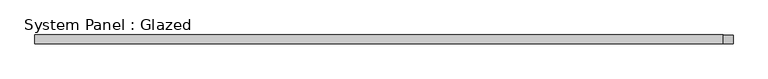
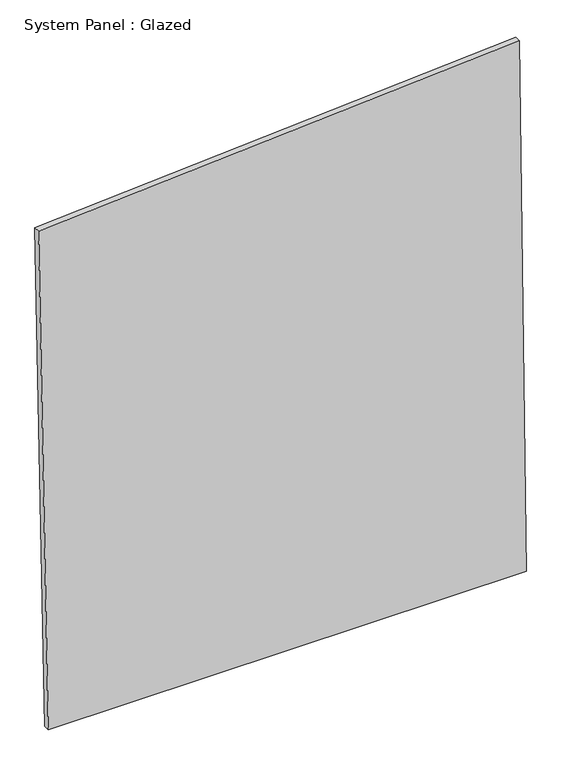
"""IFC4 building model written with IfcOpenShell, lengths in millimetres: plate geometry, System Panel : Glazed."""

from ifc_helpers import new_model, si_unit, frame, origin, place, context, project, spatial, polyline, outline, extrude, source, transform, mapped, element, save


def system_panel_glazed_7d8b04ef(model_context):
    return source(origin(), model_context, "Body", "SweptSolid", [
        extrude(outline(polyline([(0.0, -937.8383573), (0.0, 976.8018413), (2255.477521, 949.9625368), (2123.3255208, -976.8018413), (0.0, -937.8383573)])), frame((0.0, -49.5, 0.0), z_axis=(0.0, 1.0, 0.0), x_axis=(0.0, 0.0, 1.0)), (0.0, 0.0, 1.0), 25.0),
    ])


if __name__ == "__main__":
    model = new_model("IFC4")
    model_context = context("Model", 3, world=origin())
    ifc_project = project(units=[si_unit("LENGTHUNIT", "METRE", prefix="MILLI")], contexts=[model_context])
    site = spatial("IfcSite", under=ifc_project)
    building = spatial("IfcBuilding", under=site)
    placement = place(None, origin())
    system_panel_glazed_shape = system_panel_glazed_7d8b04ef(model_context)
    element("IfcPlate", 1, ObjectType="System Panel : Glazed", at=placement, inside=building, context=model_context, shape_type="MappedRepresentation", body=[
        mapped(system_panel_glazed_shape, transform((0.0, 0.0, 0.0), x_axis=(1.0, 0.0, 0.0), y_axis=(0.0, 1.0, 0.0), z_axis=(0.0, 0.0, 1.0))),
    ])
    save(model, "model.ifc")

# Revit data of these elements
# Element 1 (IfcPlate, "System Panel : Glazed")
#   Materials on its faces: "Glass, Clear Glazing"
# Materials
#   "Glass, Clear Glazing": class "Glass", colour RGB 247 249 248, transparency 0.85, Description = "Clear glazing", Cost = 0
